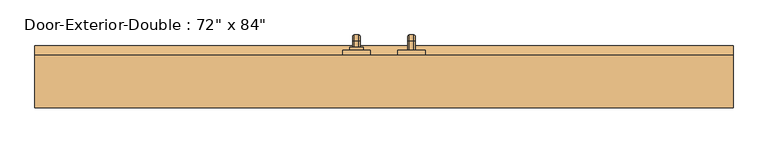
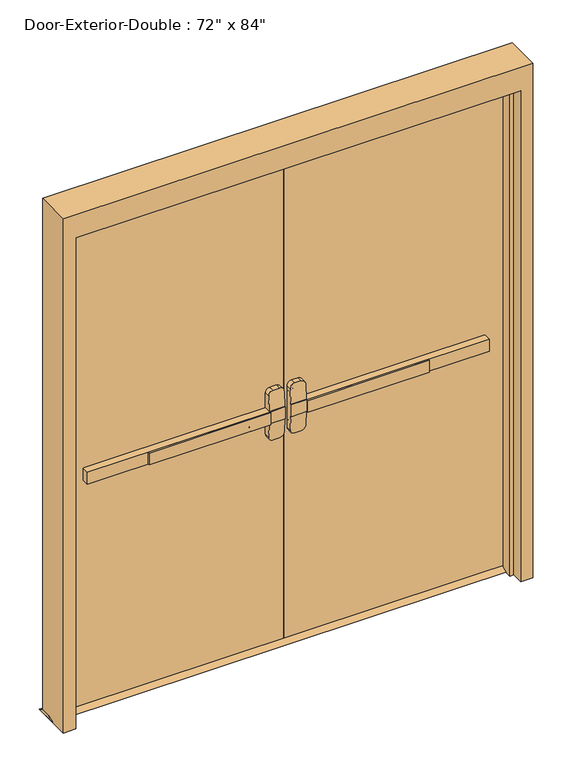
"""IFC4 building model written with IfcOpenShell, lengths in millimetres: door geometry."""

from ifc_helpers import new_model, si_unit, point, frame, frame_2d, origin, place, context, project, spatial, polyline, circle_curve, ellipse_curve, trimmed, segment, composite_curve, outline, extrude, faceted_brep, source, transform, mapped, element, save
from ifc_brep_helpers import plane_surface, cylinder_surface, revolved_surface, advanced_brep


def door_338a3df2(model_context):
    return source(origin(), model_context, "Body", "SolidModel", [
        extrude(outline(polyline([(-575.7333333, 11.1125), (-575.7333333, 17.4625), (-76.2, 17.4625), (-76.2, 11.1125), (-575.7333333, 11.1125)])), frame((0.0, 0.0, 990.6), z_axis=(0.0, 0.0, 1.0), x_axis=(1.0, 0.0, 0.0)), (0.0, 0.0, 1.0), 50.8),
        advanced_brep(
        [(-12.7, 17.4625, 1041.4), (-76.2, 17.4625, 1041.4), (-825.5, 17.4625, 1041.4), (-825.5, 17.4625, 990.6), (-76.2, 17.4625, 990.6), (-12.7, 17.4625, 990.6), (-825.5, 49.2125, 1041.4), (-76.2, 49.2125, 1041.4), (-76.2, 49.2125, 1104.9), (-57.15, 49.2125, 1123.95), (-31.75, 49.2125, 1123.95), (-12.7, 49.2125, 1104.9), (-12.7, 49.2125, 927.1), (-31.75, 49.2125, 908.05), (-57.15, 49.2125, 908.05), (-76.2, 49.2125, 927.1), (-76.2, 49.2125, 990.6), (-825.5, 49.2125, 990.6), (-12.7, 20.6377467, 1041.4), (-76.2, 20.6377467, 1041.4), (-12.7, 20.6377467, 990.6), (-12.7, 25.6479269, 927.1), (-12.7, 25.6479269, 1104.9), (-76.2, 20.6377467, 990.6), (-76.2, 25.6479269, 1104.9), (-76.2, 25.6479269, 927.1), (-57.15, 27.150981, 1123.95), (-31.75, 27.150981, 1123.95), (-31.75, 27.150981, 908.05), (-57.15, 27.150981, 908.05)],
        [
            (0, 1),
            (1, 2),
            (2, 3),
            (3, 4),
            (4, 5),
            (5, 0),
            (6, 7),
            (7, 8),
            (8, 9, circle_curve(frame((-57.15, 49.2125, 1104.9), z_axis=(0.0, 1.0, 0.0), x_axis=(-1.0, 0.0, 0.0)), 19.05)),
            (9, 10),
            (10, 11, circle_curve(frame((-31.75, 49.2125, 1104.9), z_axis=(0.0, 1.0, 0.0), x_axis=(-1.0, 0.0, 0.0)), 19.05)),
            (11, 12),
            (12, 13, circle_curve(frame((-31.75, 49.2125, 927.1), z_axis=(0.0, 1.0, 0.0), x_axis=(-1.0, 0.0, 0.0)), 19.05)),
            (13, 14),
            (14, 15, circle_curve(frame((-57.15, 49.2125, 927.1), z_axis=(0.0, 1.0, 0.0), x_axis=(-1.0, 0.0, 0.0)), 19.05)),
            (15, 16),
            (16, 17),
            (17, 6),
            (0, 18),
            (18, 19),
            (19, 7),
            (6, 2),
            (5, 20),
            (20, 21),
            (21, 12),
            (11, 22),
            (22, 18),
            (16, 23),
            (23, 20),
            (3, 17),
            (19, 24),
            (24, 8),
            (15, 25),
            (25, 23),
            (9, 26),
            (26, 27),
            (27, 10),
            (13, 28),
            (28, 29),
            (29, 14),
            (29, 25, ellipse_curve(frame((-57.15, 25.6479269, 927.1), z_axis=(0.0, 0.9969018152893365, 0.07865602756830282), x_axis=(0.0, -0.07865602756830208, 0.9969018152893365)), 19.1092038, 19.05)),
            (24, 26, ellipse_curve(frame((-57.15, 25.6479269, 1104.9), z_axis=(0.0, 0.9969018152893376, -0.07865602756828934), x_axis=(0.0, -0.078656027568288, -0.9969018152893377)), 19.1092038, 19.05)),
            (27, 22, ellipse_curve(frame((-31.75, 25.6479269, 1104.9), z_axis=(0.0, 0.9969018152893376, -0.07865602756828934), x_axis=(0.0, -0.078656027568288, -0.9969018152893377)), 19.1092038, 19.05)),
            (21, 28, ellipse_curve(frame((-31.75, 25.6479269, 927.1), z_axis=(0.0, 0.9969018152893365, 0.07865602756830282), x_axis=(0.0, -0.07865602756830208, 0.9969018152893365)), 19.1092038, 19.05)),
        ],
        [
            plane_surface(frame((-12.7, 17.4625, 1041.4), z_axis=(0.0, -1.0, 0.0), x_axis=(1.0, 0.0, 0.0))),
            plane_surface(frame((-12.7, 49.2125, 1041.4), z_axis=(0.0, 1.0, 0.0), x_axis=(-1.0, 0.0, 0.0))),
            plane_surface(frame((-825.5, 17.4625, 1041.4), z_axis=(0.0, 0.0, 1.0), x_axis=(0.0, 1.0, 0.0))),
            plane_surface(frame((-12.7, 17.4625, 1041.4), z_axis=(1.0, 0.0, 0.0), x_axis=(0.0, 1.0, 0.0))),
            plane_surface(frame((-12.7, 17.4625, 990.6), z_axis=(0.0, 0.0, -1.0), x_axis=(0.0, 1.0, 0.0))),
            plane_surface(frame((-825.5, 17.4625, 990.6), z_axis=(-1.0, 0.0, 0.0), x_axis=(0.0, 1.0, 0.0))),
            plane_surface(frame((-76.2, 20.6377467, 927.1), z_axis=(-1.0, 0.0, 0.0), x_axis=(0.0, 1.0, 0.0))),
            plane_surface(frame((-57.15, 20.6377467, 1123.95), z_axis=(0.0, 0.0, 1.0), x_axis=(0.0, 1.0, 0.0))),
            plane_surface(frame((-31.75, 20.6377467, 908.05), z_axis=(0.0, 0.0, -1.0), x_axis=(0.0, 1.0, 0.0))),
            cylinder_surface(frame((-57.15, 49.2125, 927.1), z_axis=(0.0, -1.0, 0.0), x_axis=(-1.0, 0.0, 0.0)), 19.05),
            cylinder_surface(frame((-57.15, 49.2125, 1104.9), z_axis=(0.0, -1.0, 0.0), x_axis=(-1.0, 0.0, 0.0)), 19.05),
            cylinder_surface(frame((-31.75, 49.2125, 1104.9), z_axis=(0.0, -1.0, 0.0), x_axis=(-1.0, 0.0, 0.0)), 19.05),
            cylinder_surface(frame((-31.75, 49.2125, 927.1), z_axis=(0.0, -1.0, 0.0), x_axis=(-1.0, 0.0, 0.0)), 19.05),
            plane_surface(frame((-76.2, 20.6377467, 1041.4), z_axis=(0.0, -0.9969018152893376, 0.07865602756828934), x_axis=(1.0, 0.0, 0.0))),
            plane_surface(frame((-76.2, 27.150981, 908.05), z_axis=(0.0, -0.9969018152893365, -0.07865602756830282), x_axis=(1.0, 0.0, 0.0))),
        ],
        [
            (0, [[1, 2, 3, 4, 5, 6]]),
            (1, [[7, 8, 9, 10, 11, 12, 13, 14, 15, 16, 17, 18]]),
            (2, [[-2, -1, 19, 20, 21, -7, 22]]),
            (3, [[23, 24, 25, -12, 26, 27, -19, -6]]),
            (4, [[-17, 28, 29, -23, -5, -4, 30]]),
            (5, [[-22, -18, -30, -3]]),
            (6, [[-21, 31, 32, -8]]),
            (6, [[33, 34, -28, -16]]),
            (7, [[35, 36, 37, -10]]),
            (8, [[38, 39, 40, -14]]),
            (9, [[-40, 41, -33, -15]]),
            (10, [[-32, 42, -35, -9]]),
            (11, [[-37, 43, -26, -11]]),
            (12, [[-25, 44, -38, -13]]),
            (13, [[-27, -43, -36, -42, -31, -20]]),
            (14, [[-29, -34, -41, -39, -44, -24]]),
        ],
    ),
        extrude(outline(polyline([(93.6625, 12.7), (119.0625, 0.0), (23.8125, 0.0), (49.2125, 12.7), (93.6625, 12.7)])), frame((-965.2, 0.0, 0.0), z_axis=(1.0, 0.0, 0.0), x_axis=(0.0, 1.0, 0.0)), (0.0, 0.0, 1.0), 1930.4),
        extrude(outline(polyline([(575.7333333, 11.1125), (76.2, 11.1125), (76.2, 17.4625), (575.7333333, 17.4625), (575.7333333, 11.1125)])), frame((0.0, 0.0, 990.6), z_axis=(0.0, 0.0, 1.0), x_axis=(1.0, 0.0, 0.0)), (0.0, 0.0, 1.0), 50.8),
        advanced_brep(
        [(12.7, 17.4625, 1041.4), (12.7, 17.4625, 990.6), (76.2, 17.4625, 990.6), (825.5, 17.4625, 990.6), (825.5, 17.4625, 1041.4), (76.2, 17.4625, 1041.4), (825.5, 49.2125, 1041.4), (825.5, 49.2125, 990.6), (76.2, 49.2125, 990.6), (76.2, 49.2125, 927.1), (57.15, 49.2125, 908.05), (31.75, 49.2125, 908.05), (12.7, 49.2125, 927.1), (12.7, 49.2125, 1104.9), (31.75, 49.2125, 1123.95), (57.15, 49.2125, 1123.95), (76.2, 49.2125, 1104.9), (76.2, 49.2125, 1041.4), (76.2, 20.6377467, 1041.4), (12.7, 20.6377467, 1041.4), (12.7, 25.6479269, 1104.9), (12.7, 25.6479269, 927.1), (12.7, 20.6377467, 990.6), (76.2, 20.6377467, 990.6), (76.2, 25.6479269, 927.1), (76.2, 25.6479269, 1104.9), (31.75, 27.150981, 1123.95), (57.15, 27.150981, 1123.95), (57.15, 27.150981, 908.05), (31.75, 27.150981, 908.05)],
        [
            (0, 1),
            (1, 2),
            (2, 3),
            (3, 4),
            (4, 5),
            (5, 0),
            (6, 7),
            (7, 8),
            (8, 9),
            (9, 10, circle_curve(frame((57.15, 49.2125, 927.1), z_axis=(0.0, 1.0, 0.0), x_axis=(1.0, 0.0, 0.0)), 19.05)),
            (10, 11),
            (11, 12, circle_curve(frame((31.75, 49.2125, 927.1), z_axis=(0.0, 1.0, 0.0), x_axis=(1.0, 0.0, 0.0)), 19.05)),
            (12, 13),
            (13, 14, circle_curve(frame((31.75, 49.2125, 1104.9), z_axis=(0.0, 1.0, 0.0), x_axis=(1.0, 0.0, 0.0)), 19.05)),
            (14, 15),
            (15, 16, circle_curve(frame((57.15, 49.2125, 1104.9), z_axis=(0.0, 1.0, 0.0), x_axis=(1.0, 0.0, 0.0)), 19.05)),
            (16, 17),
            (17, 6),
            (4, 6),
            (17, 18),
            (18, 19),
            (19, 0),
            (19, 20),
            (20, 13),
            (12, 21),
            (21, 22),
            (22, 1),
            (7, 3),
            (22, 23),
            (23, 8),
            (23, 24),
            (24, 9),
            (16, 25),
            (25, 18),
            (14, 26),
            (26, 27),
            (27, 15),
            (10, 28),
            (28, 29),
            (29, 11),
            (24, 28, ellipse_curve(frame((57.15, 25.6479269, 927.1), z_axis=(0.0, 0.9969018152893365, 0.07865602756830282), x_axis=(0.0, -0.07865602756830208, 0.9969018152893365)), 19.1092038, 19.05)),
            (27, 25, ellipse_curve(frame((57.15, 25.6479269, 1104.9), z_axis=(0.0, 0.9969018152893376, -0.07865602756828934), x_axis=(0.0, -0.078656027568288, -0.9969018152893377)), 19.1092038, 19.05)),
            (20, 26, ellipse_curve(frame((31.75, 25.6479269, 1104.9), z_axis=(0.0, 0.9969018152893376, -0.07865602756828934), x_axis=(0.0, -0.078656027568288, -0.9969018152893377)), 19.1092038, 19.05)),
            (29, 21, ellipse_curve(frame((31.75, 25.6479269, 927.1), z_axis=(0.0, 0.9969018152893365, 0.07865602756830282), x_axis=(0.0, -0.07865602756830208, 0.9969018152893365)), 19.1092038, 19.05)),
        ],
        [
            plane_surface(frame((12.7, 17.4625, 1041.4), z_axis=(0.0, -1.0, 0.0), x_axis=(-1.0, 0.0, 0.0))),
            plane_surface(frame((12.7, 49.2125, 1041.4), z_axis=(0.0, 1.0, 0.0), x_axis=(1.0, 0.0, 0.0))),
            plane_surface(frame((825.5, 17.4625, 1041.4), z_axis=(0.0, 0.0, 1.0), x_axis=(0.0, 1.0, 0.0))),
            plane_surface(frame((12.7, 17.4625, 1041.4), z_axis=(-1.0, 0.0, 0.0), x_axis=(0.0, 1.0, 0.0))),
            plane_surface(frame((12.7, 17.4625, 990.6), z_axis=(0.0, 0.0, -1.0), x_axis=(0.0, 1.0, 0.0))),
            plane_surface(frame((825.5, 17.4625, 990.6), z_axis=(1.0, 0.0, 0.0), x_axis=(0.0, 1.0, 0.0))),
            plane_surface(frame((76.2, 20.6377467, 927.1), z_axis=(1.0, 0.0, 0.0), x_axis=(0.0, 1.0, 0.0))),
            plane_surface(frame((57.15, 20.6377467, 1123.95), z_axis=(0.0, 0.0, 1.0), x_axis=(0.0, 1.0, 0.0))),
            plane_surface(frame((31.75, 20.6377467, 908.05), z_axis=(0.0, 0.0, -1.0), x_axis=(0.0, 1.0, 0.0))),
            cylinder_surface(frame((57.15, 49.2125, 927.1), z_axis=(0.0, -1.0, 0.0), x_axis=(1.0, 0.0, 0.0)), 19.05),
            cylinder_surface(frame((57.15, 49.2125, 1104.9), z_axis=(0.0, -1.0, 0.0), x_axis=(1.0, 0.0, 0.0)), 19.05),
            cylinder_surface(frame((31.75, 49.2125, 1104.9), z_axis=(0.0, -1.0, 0.0), x_axis=(1.0, 0.0, 0.0)), 19.05),
            cylinder_surface(frame((31.75, 49.2125, 927.1), z_axis=(0.0, -1.0, 0.0), x_axis=(1.0, 0.0, 0.0)), 19.05),
            plane_surface(frame((76.2, 20.6377467, 1041.4), z_axis=(0.0, -0.9969018152893376, 0.07865602756828934), x_axis=(-1.0, 0.0, 0.0))),
            plane_surface(frame((76.2, 27.150981, 908.05), z_axis=(0.0, -0.9969018152893365, -0.07865602756830282), x_axis=(-1.0, 0.0, 0.0))),
        ],
        [
            (0, [[1, 2, 3, 4, 5, 6]]),
            (1, [[7, 8, 9, 10, 11, 12, 13, 14, 15, 16, 17, 18]]),
            (2, [[19, -18, 20, 21, 22, -6, -5]]),
            (3, [[-1, -22, 23, 24, -13, 25, 26, 27]]),
            (4, [[28, -3, -2, -27, 29, 30, -8]]),
            (5, [[-4, -28, -7, -19]]),
            (6, [[-9, -30, 31, 32]]),
            (6, [[-17, 33, 34, -20]]),
            (7, [[-15, 35, 36, 37]]),
            (8, [[-11, 38, 39, 40]]),
            (9, [[-10, -32, 41, -38]]),
            (10, [[-16, -37, 42, -33]]),
            (11, [[-14, -24, 43, -35]]),
            (12, [[-12, -40, 44, -25]]),
            (13, [[-21, -34, -42, -36, -43, -23]]),
            (14, [[-26, -44, -39, -41, -31, -29]]),
        ],
    ),
        advanced_brep(
        [(66.2, 106.3625, 1017.190625), (66.2, 106.3625, 1014.809375), (69.771875, 106.3625, 1011.2375), (82.6284594, 106.3625, 1011.2375), (86.2, 106.3625, 1014.8090406), (86.2, 106.3625, 1017.190625), (82.628125, 106.3625, 1020.7625), (69.771875, 106.3625, 1020.7625), (66.2, 106.3625, 887.809375), (69.771875, 106.3625, 884.2375), (82.628125, 106.3625, 884.2375), (86.2, 106.3625, 887.809375), (86.2, 106.3625, 890.1909594), (82.6284594, 106.3625, 893.7625), (69.771875, 106.3625, 893.7625), (66.2, 106.3625, 890.190625), (66.2, 131.7625, 1017.190625), (66.2, 145.653125, 1003.3), (66.2, 145.653125, 901.7), (66.2, 131.7625, 887.809375), (66.2, 131.7625, 890.190625), (66.2, 143.271875, 901.7), (66.2, 143.271875, 1003.3), (66.2, 131.7625, 1014.809375), (69.771875, 131.7625, 1011.2375), (82.6284594, 131.7625, 1011.2375), (86.2, 131.7625, 1014.8090406), (86.2, 143.2715406, 1003.3), (86.2, 143.2715406, 901.7), (86.2, 131.7625, 890.1909594), (86.2, 131.7625, 887.809375), (86.2, 145.653125, 901.7), (86.2, 145.653125, 1003.3), (86.2, 131.7625, 1017.190625), (82.628125, 131.7625, 1020.7625), (69.771875, 131.7625, 1020.7625), (69.771875, 139.7, 1003.3), (82.6284594, 139.7, 1003.3), (82.628125, 149.225, 1003.3), (69.771875, 149.225, 1003.3), (69.771875, 139.7, 901.7), (82.6284594, 139.7, 901.7), (82.628125, 149.225, 901.7), (69.771875, 149.225, 901.7), (69.771875, 131.7625, 893.7625), (82.6284594, 131.7625, 893.7625), (82.628125, 131.7625, 884.2375), (69.771875, 131.7625, 884.2375)],
        [
            (0, 1),
            (1, 2, circle_curve(frame((69.771875, 106.3625, 1014.809375), z_axis=(0.0, -1.0, 0.0), x_axis=(0.0, 0.0, 1.0)), 3.571875)),
            (2, 3),
            (3, 4, circle_curve(frame((82.6284594, 106.3625, 1014.8090406), z_axis=(0.0, -1.0, 0.0), x_axis=(0.0, 0.0, 1.0)), 3.5715406)),
            (4, 5),
            (5, 6, circle_curve(frame((82.628125, 106.3625, 1017.190625), z_axis=(0.0, -1.0, 0.0), x_axis=(0.0, 0.0, 1.0)), 3.571875)),
            (6, 7),
            (7, 0, circle_curve(frame((69.771875, 106.3625, 1017.190625), z_axis=(0.0, -1.0, 0.0), x_axis=(0.0, 0.0, 1.0)), 3.571875)),
            (8, 9, circle_curve(frame((69.771875, 106.3625, 887.809375), z_axis=(0.0, -1.0, 0.0), x_axis=(0.0, 0.0, -1.0)), 3.571875)),
            (9, 10),
            (10, 11, circle_curve(frame((82.628125, 106.3625, 887.809375), z_axis=(0.0, -1.0, 0.0), x_axis=(0.0, 0.0, -1.0)), 3.571875)),
            (11, 12),
            (12, 13, circle_curve(frame((82.6284594, 106.3625, 890.1909594), z_axis=(0.0, -1.0, 0.0), x_axis=(0.0, 0.0, -1.0)), 3.5715406)),
            (13, 14),
            (14, 15, circle_curve(frame((69.771875, 106.3625, 890.190625), z_axis=(0.0, -1.0, 0.0), x_axis=(0.0, 0.0, -1.0)), 3.571875)),
            (15, 8),
            (0, 16),
            (16, 17, circle_curve(frame((66.2, 131.7625, 1003.3), z_axis=(-1.0, 0.0, 0.0), x_axis=(0.0, 0.0, 1.0)), 13.890625)),
            (17, 18),
            (18, 19, circle_curve(frame((66.2, 131.7625, 901.7), z_axis=(-1.0, 0.0, 0.0), x_axis=(0.0, 1.0, 0.0)), 13.890625)),
            (19, 8),
            (15, 20),
            (20, 21, circle_curve(frame((66.2, 131.7625, 901.7), z_axis=(1.0, 0.0, 0.0), x_axis=(0.0, 1.0, 0.0)), 11.509375)),
            (21, 22),
            (22, 23, circle_curve(frame((66.2, 131.7625, 1003.3), z_axis=(1.0, 0.0, 0.0), x_axis=(0.0, 0.0, 1.0)), 11.509375)),
            (23, 1),
            (23, 24, circle_curve(frame((69.771875, 131.7625, 1014.809375), z_axis=(0.0, -1.0, 0.0), x_axis=(0.0, 0.0, 1.0)), 3.571875)),
            (24, 2),
            (24, 25),
            (25, 3),
            (25, 26, circle_curve(frame((82.6284594, 131.7625, 1014.8090406), z_axis=(0.0, -1.0, 0.0), x_axis=(0.0, 0.0, 1.0)), 3.5715406)),
            (26, 4),
            (26, 27, circle_curve(frame((86.2, 131.7625, 1003.3), z_axis=(-1.0, 0.0, 0.0), x_axis=(0.0, 0.0, 1.0)), 11.5090406)),
            (27, 28),
            (28, 29, circle_curve(frame((86.2, 131.7625, 901.7), z_axis=(-1.0, 0.0, 0.0), x_axis=(0.0, 1.0, 0.0)), 11.5090406)),
            (29, 12),
            (11, 30),
            (30, 31, circle_curve(frame((86.2, 131.7625, 901.7), z_axis=(1.0, 0.0, 0.0), x_axis=(0.0, 1.0, 0.0)), 13.890625)),
            (31, 32),
            (32, 33, circle_curve(frame((86.2, 131.7625, 1003.3), z_axis=(1.0, 0.0, 0.0), x_axis=(0.0, 0.0, 1.0)), 13.890625)),
            (33, 5),
            (33, 34, circle_curve(frame((82.628125, 131.7625, 1017.190625), z_axis=(0.0, -1.0, 0.0), x_axis=(0.0, 0.0, 1.0)), 3.571875)),
            (34, 6),
            (34, 35),
            (35, 7),
            (35, 16, circle_curve(frame((69.771875, 131.7625, 1017.190625), z_axis=(0.0, -1.0, 0.0), x_axis=(0.0, 0.0, 1.0)), 3.571875)),
            (36, 24, circle_curve(frame((69.771875, 131.7625, 1003.3), z_axis=(1.0, 0.0, 0.0), x_axis=(0.0, 0.0, 1.0)), 7.9375)),
            (22, 36, circle_curve(frame((69.771875, 143.271875, 1003.3), z_axis=(0.0, 0.0, 1.0), x_axis=(0.0, 1.0, 0.0)), 3.571875)),
            (37, 25, circle_curve(frame((82.6284594, 131.7625, 1003.3), z_axis=(1.0, 0.0, 0.0), x_axis=(0.0, 0.0, 1.0)), 7.9375)),
            (36, 37),
            (37, 27, circle_curve(frame((82.6284594, 143.2715406, 1003.3), z_axis=(0.0, 0.0, 1.0), x_axis=(0.0, 1.0, 0.0)), 3.5715406)),
            (38, 34, circle_curve(frame((82.628125, 131.7625, 1003.3), z_axis=(1.0, 0.0, 0.0), x_axis=(0.0, 0.0, 1.0)), 17.4625)),
            (32, 38, circle_curve(frame((82.628125, 145.653125, 1003.3), z_axis=(0.0, 0.0, 1.0), x_axis=(0.0, 1.0, 0.0)), 3.571875)),
            (39, 35, circle_curve(frame((69.771875, 131.7625, 1003.3), z_axis=(1.0, 0.0, 0.0), x_axis=(0.0, 0.0, 1.0)), 17.4625)),
            (38, 39),
            (39, 17, circle_curve(frame((69.771875, 145.653125, 1003.3), z_axis=(0.0, 0.0, 1.0), x_axis=(0.0, 1.0, 0.0)), 3.571875)),
            (21, 40, circle_curve(frame((69.771875, 143.271875, 901.7), z_axis=(0.0, 0.0, 1.0), x_axis=(0.0, 1.0, 0.0)), 3.571875)),
            (40, 36),
            (40, 41),
            (41, 37),
            (41, 28, circle_curve(frame((82.6284594, 143.2715406, 901.7), z_axis=(0.0, 0.0, 1.0), x_axis=(0.0, 1.0, 0.0)), 3.5715406)),
            (31, 42, circle_curve(frame((82.628125, 145.653125, 901.7), z_axis=(0.0, 0.0, 1.0), x_axis=(0.0, 1.0, 0.0)), 3.571875)),
            (42, 38),
            (42, 43),
            (43, 39),
            (43, 18, circle_curve(frame((69.771875, 145.653125, 901.7), z_axis=(0.0, 0.0, 1.0), x_axis=(0.0, 1.0, 0.0)), 3.571875)),
            (44, 40, circle_curve(frame((69.771875, 131.7625, 901.7), z_axis=(1.0, 0.0, 0.0), x_axis=(0.0, 1.0, 0.0)), 7.9375)),
            (20, 44, circle_curve(frame((69.771875, 131.7625, 890.190625), z_axis=(0.0, 1.0, 0.0), x_axis=(0.0, 0.0, -1.0)), 3.571875)),
            (45, 41, circle_curve(frame((82.6284594, 131.7625, 901.7), z_axis=(1.0, 0.0, 0.0), x_axis=(0.0, 1.0, 0.0)), 7.9375)),
            (44, 45),
            (45, 29, circle_curve(frame((82.6284594, 131.7625, 890.1909594), z_axis=(0.0, 1.0, 0.0), x_axis=(0.0, 0.0, -1.0)), 3.5715406)),
            (46, 42, circle_curve(frame((82.628125, 131.7625, 901.7), z_axis=(1.0, 0.0, 0.0), x_axis=(0.0, 1.0, 0.0)), 17.4625)),
            (30, 46, circle_curve(frame((82.628125, 131.7625, 887.809375), z_axis=(0.0, 1.0, 0.0), x_axis=(0.0, 0.0, -1.0)), 3.571875)),
            (47, 43, circle_curve(frame((69.771875, 131.7625, 901.7), z_axis=(1.0, 0.0, 0.0), x_axis=(0.0, 1.0, 0.0)), 17.4625)),
            (46, 47),
            (47, 19, circle_curve(frame((69.771875, 131.7625, 887.809375), z_axis=(0.0, 1.0, 0.0), x_axis=(0.0, 0.0, -1.0)), 3.571875)),
            (14, 44),
            (13, 45),
            (10, 46),
            (9, 47),
        ],
        [
            plane_surface(frame((76.2, 106.3625, 1016.0), z_axis=(0.0, -1.0, 0.0), x_axis=(1.0, 0.0, 0.0))),
            plane_surface(frame((76.2, 106.3625, 889.0), z_axis=(0.0, -1.0, 0.0), x_axis=(1.0, 0.0, 0.0))),
            plane_surface(frame((66.2, 106.3625, 1017.190625), z_axis=(-1.0, 0.0, 0.0), x_axis=(0.0, 1.0, 0.0))),
            cylinder_surface(frame((69.771875, 106.3625, 1014.809375), z_axis=(0.0, -1.0, 0.0), x_axis=(0.0, 0.0, 1.0)), 3.571875),
            plane_surface(frame((69.771875, 106.3625, 1011.2375), z_axis=(0.0, 0.0, -1.0), x_axis=(0.0, 1.0, 0.0))),
            cylinder_surface(frame((82.6284594, 106.3625, 1014.8090406), z_axis=(0.0, -1.0, 0.0), x_axis=(0.0, 0.0, 1.0)), 3.5715406),
            plane_surface(frame((86.2, 106.3625, 1014.8090406), z_axis=(1.0, 0.0, 0.0), x_axis=(0.0, 1.0, 0.0))),
            cylinder_surface(frame((82.628125, 106.3625, 1017.190625), z_axis=(0.0, -1.0, 0.0), x_axis=(0.0, 0.0, 1.0)), 3.571875),
            plane_surface(frame((82.628125, 106.3625, 1020.7625), z_axis=(0.0, 0.0, 1.0), x_axis=(0.0, 1.0, 0.0))),
            cylinder_surface(frame((69.771875, 106.3625, 1017.190625), z_axis=(0.0, -1.0, 0.0), x_axis=(0.0, 0.0, 1.0)), 3.571875),
            revolved_surface(trimmed(ellipse_curve(frame((69.771875, 131.7625, 1014.809375), z_axis=(0.0, -1.0, 0.0), x_axis=(0.0, 0.0, 1.0)), 3.571875, 3.571875), [point((66.2, 131.7625, 1014.809375))], [point((69.771875, 131.7625, 1011.2375))], True, "CARTESIAN"), (76.2, 131.7625, 1003.3), (-1.0, 0.0, 0.0)),
            revolved_surface(polyline([(69.771875, 131.7625, 1011.2375), (82.6284594, 131.7625, 1011.2375)]), (76.2, 131.7625, 1003.3), (-1.0, 0.0, 0.0)),
            revolved_surface(trimmed(ellipse_curve(frame((82.6284594, 131.7625, 1014.8090406), z_axis=(0.0, -1.0, 0.0), x_axis=(0.0, 0.0, 1.0)), 3.5715406, 3.5715406), [point((82.6284594, 131.7625, 1011.2375))], [point((86.2, 131.7625, 1014.8090406))], True, "CARTESIAN"), (76.2, 131.7625, 1003.3), (-1.0, 0.0, 0.0)),
            revolved_surface(trimmed(ellipse_curve(frame((82.628125, 131.7625, 1017.190625), z_axis=(0.0, -1.0, 0.0), x_axis=(0.0, 0.0, 1.0)), 3.571875, 3.571875), [point((86.2, 131.7625, 1017.190625))], [point((82.628125, 131.7625, 1020.7625))], True, "CARTESIAN"), (76.2, 131.7625, 1003.3), (-1.0, 0.0, 0.0)),
            cylinder_surface(frame((76.2, 131.7625, 1003.3), z_axis=(-1.0, 0.0, 0.0), x_axis=(0.0, 0.0, 1.0)), 17.4625),
            revolved_surface(trimmed(ellipse_curve(frame((69.771875, 131.7625, 1017.190625), z_axis=(0.0, -1.0, 0.0), x_axis=(0.0, 0.0, 1.0)), 3.571875, 3.571875), [point((69.771875, 131.7625, 1020.7625))], [point((66.2, 131.7625, 1017.190625))], True, "CARTESIAN"), (76.2, 131.7625, 1003.3), (-1.0, 0.0, 0.0)),
            cylinder_surface(frame((69.771875, 143.271875, 1003.3), z_axis=(0.0, 0.0, 1.0), x_axis=(0.0, 1.0, 0.0)), 3.571875),
            plane_surface(frame((69.771875, 139.7, 1003.3), z_axis=(0.0, -1.0, 0.0), x_axis=(0.0, 0.0, -1.0))),
            cylinder_surface(frame((82.6284594, 143.2715406, 1003.3), z_axis=(0.0, 0.0, 1.0), x_axis=(0.0, 1.0, 0.0)), 3.5715406),
            cylinder_surface(frame((82.628125, 145.653125, 1003.3), z_axis=(0.0, 0.0, 1.0), x_axis=(0.0, 1.0, 0.0)), 3.571875),
            plane_surface(frame((82.628125, 149.225, 1003.3), z_axis=(0.0, 1.0, 0.0), x_axis=(0.0, 0.0, -1.0))),
            cylinder_surface(frame((69.771875, 145.653125, 1003.3), z_axis=(0.0, 0.0, 1.0), x_axis=(0.0, 1.0, 0.0)), 3.571875),
            revolved_surface(trimmed(ellipse_curve(frame((69.771875, 143.271875, 901.7), z_axis=(0.0, 0.0, 1.0), x_axis=(0.0, 1.0, 0.0)), 3.571875, 3.571875), [point((66.2, 143.271875, 901.7))], [point((69.771875, 139.7, 901.7))], True, "CARTESIAN"), (76.2, 131.7625, 901.7), (-1.0, 0.0, 0.0)),
            revolved_surface(polyline([(69.771875, 139.7, 901.7), (82.6284594, 139.7, 901.7)]), (76.2, 131.7625, 901.7), (-1.0, 0.0, 0.0)),
            revolved_surface(trimmed(ellipse_curve(frame((82.6284594, 143.2715406, 901.7), z_axis=(0.0, 0.0, 1.0), x_axis=(0.0, 1.0, 0.0)), 3.5715406, 3.5715406), [point((82.6284594, 139.7, 901.7))], [point((86.2, 143.2715406, 901.7))], True, "CARTESIAN"), (76.2, 131.7625, 901.7), (-1.0, 0.0, 0.0)),
            revolved_surface(trimmed(ellipse_curve(frame((82.628125, 145.653125, 901.7), z_axis=(0.0, 0.0, 1.0), x_axis=(0.0, 1.0, 0.0)), 3.571875, 3.571875), [point((86.2, 145.653125, 901.7))], [point((82.628125, 149.225, 901.7))], True, "CARTESIAN"), (76.2, 131.7625, 901.7), (-1.0, 0.0, 0.0)),
            cylinder_surface(frame((76.2, 131.7625, 901.7), z_axis=(-1.0, 0.0, 0.0), x_axis=(0.0, 1.0, 0.0)), 17.4625),
            revolved_surface(trimmed(ellipse_curve(frame((69.771875, 145.653125, 901.7), z_axis=(0.0, 0.0, 1.0), x_axis=(0.0, 1.0, 0.0)), 3.571875, 3.571875), [point((69.771875, 149.225, 901.7))], [point((66.2, 145.653125, 901.7))], True, "CARTESIAN"), (76.2, 131.7625, 901.7), (-1.0, 0.0, 0.0)),
            cylinder_surface(frame((69.771875, 131.7625, 890.190625), z_axis=(0.0, 1.0, 0.0), x_axis=(0.0, 0.0, -1.0)), 3.571875),
            plane_surface(frame((69.771875, 131.7625, 893.7625), z_axis=(0.0, 0.0, 1.0), x_axis=(0.0, -1.0, 0.0))),
            cylinder_surface(frame((82.6284594, 131.7625, 890.1909594), z_axis=(0.0, 1.0, 0.0), x_axis=(0.0, 0.0, -1.0)), 3.5715406),
            cylinder_surface(frame((82.628125, 131.7625, 887.809375), z_axis=(0.0, 1.0, 0.0), x_axis=(0.0, 0.0, -1.0)), 3.571875),
            plane_surface(frame((82.628125, 131.7625, 884.2375), z_axis=(0.0, 0.0, -1.0), x_axis=(0.0, -1.0, 0.0))),
            cylinder_surface(frame((69.771875, 131.7625, 887.809375), z_axis=(0.0, 1.0, 0.0), x_axis=(0.0, 0.0, -1.0)), 3.571875),
        ],
        [
            (0, [[1, 2, 3, 4, 5, 6, 7, 8]]),
            (1, [[9, 10, 11, 12, 13, 14, 15, 16]]),
            (2, [[-1, 17, 18, 19, 20, 21, -16, 22, 23, 24, 25, 26]]),
            (3, [[-2, -26, 27, 28]]),
            (4, [[-3, -28, 29, 30]]),
            (5, [[-4, -30, 31, 32]]),
            (6, [[-5, -32, 33, 34, 35, 36, -12, 37, 38, 39, 40, 41]]),
            (7, [[-6, -41, 42, 43]]),
            (8, [[-7, -43, 44, 45]]),
            (9, [[-8, -45, 46, -17]]),
            (10, [[47, -27, -25, 48]]),
            (11, [[49, -29, -47, 50]]),
            (12, [[-33, -31, -49, 51]]),
            (13, [[52, -42, -40, 53]]),
            (14, [[54, -44, -52, 55]]),
            (15, [[-18, -46, -54, 56]]),
            (16, [[-48, -24, 57, 58]]),
            (17, [[-50, -58, 59, 60]]),
            (18, [[-51, -60, 61, -34]]),
            (19, [[-53, -39, 62, 63]]),
            (20, [[-55, -63, 64, 65]]),
            (21, [[-56, -65, 66, -19]]),
            (22, [[67, -57, -23, 68]]),
            (23, [[69, -59, -67, 70]]),
            (24, [[-35, -61, -69, 71]]),
            (25, [[72, -62, -38, 73]]),
            (26, [[74, -64, -72, 75]]),
            (27, [[-20, -66, -74, 76]]),
            (28, [[-68, -22, -15, 77]]),
            (29, [[-70, -77, -14, 78]]),
            (30, [[-71, -78, -13, -36]]),
            (31, [[-73, -37, -11, 79]]),
            (32, [[-75, -79, -10, 80]]),
            (33, [[-76, -80, -9, -21]]),
        ],
    ),
        extrude(outline(composite_curve([segment(trimmed(circle_curve(frame_2d((1113.0338574, 76.2)), 89.3016225), [point((1193.8, 114.3))], [point((1193.8, 38.1))], False, "CARTESIAN"), True, "CONTINUOUS"), segment(polyline([(1193.8, 38.1), (838.2, 38.1)]), True, "CONTINUOUS"), segment(trimmed(circle_curve(frame_2d((918.9661426, 76.2)), 89.3016225), [point((838.2, 38.1))], [point((838.2, 114.3))], False, "CARTESIAN"), True, "CONTINUOUS"), segment(polyline([(838.2, 114.3), (1193.8, 114.3)]), True, "CONTINUOUS")], self_intersect=False)), frame((0.0, 93.6625, 0.0), z_axis=(0.0, 1.0, 0.0), x_axis=(0.0, 0.0, 1.0)), (0.0, 0.0, 1.0), 12.7),
        advanced_brep(
        [(-86.2, 106.3625, 1017.190625), (-86.2, 106.3625, 1014.809375), (-82.628125, 106.3625, 1011.2375), (-69.7715406, 106.3625, 1011.2375), (-66.2, 106.3625, 1014.8090406), (-66.2, 106.3625, 1017.190625), (-69.771875, 106.3625, 1020.7625), (-82.628125, 106.3625, 1020.7625), (-86.2, 106.3625, 887.809375), (-82.628125, 106.3625, 884.2375), (-69.771875, 106.3625, 884.2375), (-66.2, 106.3625, 887.809375), (-66.2, 106.3625, 890.1909594), (-69.7715406, 106.3625, 893.7625), (-82.628125, 106.3625, 893.7625), (-86.2, 106.3625, 890.190625), (-86.2, 131.7625, 1017.190625), (-86.2, 145.653125, 1003.3), (-86.2, 145.653125, 901.7), (-86.2, 131.7625, 887.809375), (-86.2, 131.7625, 890.190625), (-86.2, 143.271875, 901.7), (-86.2, 143.271875, 1003.3), (-86.2, 131.7625, 1014.809375), (-82.628125, 131.7625, 1011.2375), (-69.7715406, 131.7625, 1011.2375), (-66.2, 131.7625, 1014.8090406), (-66.2, 143.2715406, 1003.3), (-66.2, 143.2715406, 901.7), (-66.2, 131.7625, 890.1909594), (-66.2, 131.7625, 887.809375), (-66.2, 145.653125, 901.7), (-66.2, 145.653125, 1003.3), (-66.2, 131.7625, 1017.190625), (-69.771875, 131.7625, 1020.7625), (-82.628125, 131.7625, 1020.7625), (-82.628125, 139.7, 1003.3), (-69.7715406, 139.7, 1003.3), (-69.771875, 149.225, 1003.3), (-82.628125, 149.225, 1003.3), (-82.628125, 139.7, 901.7), (-69.7715406, 139.7, 901.7), (-69.771875, 149.225, 901.7), (-82.628125, 149.225, 901.7), (-82.628125, 131.7625, 893.7625), (-69.7715406, 131.7625, 893.7625), (-69.771875, 131.7625, 884.2375), (-82.628125, 131.7625, 884.2375)],
        [
            (0, 1),
            (1, 2, circle_curve(frame((-82.628125, 106.3625, 1014.809375), z_axis=(0.0, -1.0, 0.0), x_axis=(0.0, 0.0, 1.0)), 3.571875)),
            (2, 3),
            (3, 4, circle_curve(frame((-69.7715406, 106.3625, 1014.8090406), z_axis=(0.0, -1.0, 0.0), x_axis=(0.0, 0.0, 1.0)), 3.5715406)),
            (4, 5),
            (5, 6, circle_curve(frame((-69.771875, 106.3625, 1017.190625), z_axis=(0.0, -1.0, 0.0), x_axis=(0.0, 0.0, 1.0)), 3.571875)),
            (6, 7),
            (7, 0, circle_curve(frame((-82.628125, 106.3625, 1017.190625), z_axis=(0.0, -1.0, 0.0), x_axis=(0.0, 0.0, 1.0)), 3.571875)),
            (8, 9, circle_curve(frame((-82.628125, 106.3625, 887.809375), z_axis=(0.0, -1.0, 0.0), x_axis=(0.0, 0.0, -1.0)), 3.571875)),
            (9, 10),
            (10, 11, circle_curve(frame((-69.771875, 106.3625, 887.809375), z_axis=(0.0, -1.0, 0.0), x_axis=(0.0, 0.0, -1.0)), 3.571875)),
            (11, 12),
            (12, 13, circle_curve(frame((-69.7715406, 106.3625, 890.1909594), z_axis=(0.0, -1.0, 0.0), x_axis=(0.0, 0.0, -1.0)), 3.5715406)),
            (13, 14),
            (14, 15, circle_curve(frame((-82.628125, 106.3625, 890.190625), z_axis=(0.0, -1.0, 0.0), x_axis=(0.0, 0.0, -1.0)), 3.571875)),
            (15, 8),
            (0, 16),
            (16, 17, circle_curve(frame((-86.2, 131.7625, 1003.3), z_axis=(-1.0, 0.0, 0.0), x_axis=(0.0, 0.0, 1.0)), 13.890625)),
            (17, 18),
            (18, 19, circle_curve(frame((-86.2, 131.7625, 901.7), z_axis=(-1.0, 0.0, 0.0), x_axis=(0.0, 1.0, 0.0)), 13.890625)),
            (19, 8),
            (15, 20),
            (20, 21, circle_curve(frame((-86.2, 131.7625, 901.7), z_axis=(1.0, 0.0, 0.0), x_axis=(0.0, 1.0, 0.0)), 11.509375)),
            (21, 22),
            (22, 23, circle_curve(frame((-86.2, 131.7625, 1003.3), z_axis=(1.0, 0.0, 0.0), x_axis=(0.0, 0.0, 1.0)), 11.509375)),
            (23, 1),
            (23, 24, circle_curve(frame((-82.628125, 131.7625, 1014.809375), z_axis=(0.0, -1.0, 0.0), x_axis=(0.0, 0.0, 1.0)), 3.571875)),
            (24, 2),
            (24, 25),
            (25, 3),
            (25, 26, circle_curve(frame((-69.7715406, 131.7625, 1014.8090406), z_axis=(0.0, -1.0, 0.0), x_axis=(0.0, 0.0, 1.0)), 3.5715406)),
            (26, 4),
            (26, 27, circle_curve(frame((-66.2, 131.7625, 1003.3), z_axis=(-1.0, 0.0, 0.0), x_axis=(0.0, 0.0, 1.0)), 11.5090406)),
            (27, 28),
            (28, 29, circle_curve(frame((-66.2, 131.7625, 901.7), z_axis=(-1.0, 0.0, 0.0), x_axis=(0.0, 1.0, 0.0)), 11.5090406)),
            (29, 12),
            (11, 30),
            (30, 31, circle_curve(frame((-66.2, 131.7625, 901.7), z_axis=(1.0, 0.0, 0.0), x_axis=(0.0, 1.0, 0.0)), 13.890625)),
            (31, 32),
            (32, 33, circle_curve(frame((-66.2, 131.7625, 1003.3), z_axis=(1.0, 0.0, 0.0), x_axis=(0.0, 0.0, 1.0)), 13.890625)),
            (33, 5),
            (33, 34, circle_curve(frame((-69.771875, 131.7625, 1017.190625), z_axis=(0.0, -1.0, 0.0), x_axis=(0.0, 0.0, 1.0)), 3.571875)),
            (34, 6),
            (34, 35),
            (35, 7),
            (35, 16, circle_curve(frame((-82.628125, 131.7625, 1017.190625), z_axis=(0.0, -1.0, 0.0), x_axis=(0.0, 0.0, 1.0)), 3.571875)),
            (36, 24, circle_curve(frame((-82.628125, 131.7625, 1003.3), z_axis=(1.0, 0.0, 0.0), x_axis=(0.0, 0.0, 1.0)), 7.9375)),
            (22, 36, circle_curve(frame((-82.628125, 143.271875, 1003.3), z_axis=(0.0, 0.0, 1.0), x_axis=(0.0, 1.0, 0.0)), 3.571875)),
            (37, 25, circle_curve(frame((-69.7715406, 131.7625, 1003.3), z_axis=(1.0, 0.0, 0.0), x_axis=(0.0, 0.0, 1.0)), 7.9375)),
            (36, 37),
            (37, 27, circle_curve(frame((-69.7715406, 143.2715406, 1003.3), z_axis=(0.0, 0.0, 1.0), x_axis=(0.0, 1.0, 0.0)), 3.5715406)),
            (38, 34, circle_curve(frame((-69.771875, 131.7625, 1003.3), z_axis=(1.0, 0.0, 0.0), x_axis=(0.0, 0.0, 1.0)), 17.4625)),
            (32, 38, circle_curve(frame((-69.771875, 145.653125, 1003.3), z_axis=(0.0, 0.0, 1.0), x_axis=(0.0, 1.0, 0.0)), 3.571875)),
            (39, 35, circle_curve(frame((-82.628125, 131.7625, 1003.3), z_axis=(1.0, 0.0, 0.0), x_axis=(0.0, 0.0, 1.0)), 17.4625)),
            (38, 39),
            (39, 17, circle_curve(frame((-82.628125, 145.653125, 1003.3), z_axis=(0.0, 0.0, 1.0), x_axis=(0.0, 1.0, 0.0)), 3.571875)),
            (21, 40, circle_curve(frame((-82.628125, 143.271875, 901.7), z_axis=(0.0, 0.0, 1.0), x_axis=(0.0, 1.0, 0.0)), 3.571875)),
            (40, 36),
            (40, 41),
            (41, 37),
            (41, 28, circle_curve(frame((-69.7715406, 143.2715406, 901.7), z_axis=(0.0, 0.0, 1.0), x_axis=(0.0, 1.0, 0.0)), 3.5715406)),
            (31, 42, circle_curve(frame((-69.771875, 145.653125, 901.7), z_axis=(0.0, 0.0, 1.0), x_axis=(0.0, 1.0, 0.0)), 3.571875)),
            (42, 38),
            (42, 43),
            (43, 39),
            (43, 18, circle_curve(frame((-82.628125, 145.653125, 901.7), z_axis=(0.0, 0.0, 1.0), x_axis=(0.0, 1.0, 0.0)), 3.571875)),
            (44, 40, circle_curve(frame((-82.628125, 131.7625, 901.7), z_axis=(1.0, 0.0, 0.0), x_axis=(0.0, 1.0, 0.0)), 7.9375)),
            (20, 44, circle_curve(frame((-82.628125, 131.7625, 890.190625), z_axis=(0.0, 1.0, 0.0), x_axis=(0.0, 0.0, -1.0)), 3.571875)),
            (45, 41, circle_curve(frame((-69.7715406, 131.7625, 901.7), z_axis=(1.0, 0.0, 0.0), x_axis=(0.0, 1.0, 0.0)), 7.9375)),
            (44, 45),
            (45, 29, circle_curve(frame((-69.7715406, 131.7625, 890.1909594), z_axis=(0.0, 1.0, 0.0), x_axis=(0.0, 0.0, -1.0)), 3.5715406)),
            (46, 42, circle_curve(frame((-69.771875, 131.7625, 901.7), z_axis=(1.0, 0.0, 0.0), x_axis=(0.0, 1.0, 0.0)), 17.4625)),
            (30, 46, circle_curve(frame((-69.771875, 131.7625, 887.809375), z_axis=(0.0, 1.0, 0.0), x_axis=(0.0, 0.0, -1.0)), 3.571875)),
            (47, 43, circle_curve(frame((-82.628125, 131.7625, 901.7), z_axis=(1.0, 0.0, 0.0), x_axis=(0.0, 1.0, 0.0)), 17.4625)),
            (46, 47),
            (47, 19, circle_curve(frame((-82.628125, 131.7625, 887.809375), z_axis=(0.0, 1.0, 0.0), x_axis=(0.0, 0.0, -1.0)), 3.571875)),
            (14, 44),
            (13, 45),
            (10, 46),
            (9, 47),
        ],
        [
            plane_surface(frame((-76.2, 106.3625, 1016.0), z_axis=(0.0, -1.0, 0.0), x_axis=(1.0, 0.0, 0.0))),
            plane_surface(frame((-76.2, 106.3625, 889.0), z_axis=(0.0, -1.0, 0.0), x_axis=(1.0, 0.0, 0.0))),
            plane_surface(frame((-86.2, 106.3625, 1017.190625), z_axis=(-1.0, 0.0, 0.0), x_axis=(0.0, 1.0, 0.0))),
            cylinder_surface(frame((-82.628125, 106.3625, 1014.809375), z_axis=(0.0, -1.0, 0.0), x_axis=(0.0, 0.0, 1.0)), 3.571875),
            plane_surface(frame((-82.628125, 106.3625, 1011.2375), z_axis=(0.0, 0.0, -1.0), x_axis=(0.0, 1.0, 0.0))),
            cylinder_surface(frame((-69.7715406, 106.3625, 1014.8090406), z_axis=(0.0, -1.0, 0.0), x_axis=(0.0, 0.0, 1.0)), 3.5715406),
            plane_surface(frame((-66.2, 106.3625, 1014.8090406), z_axis=(1.0, 0.0, 0.0), x_axis=(0.0, 1.0, 0.0))),
            cylinder_surface(frame((-69.771875, 106.3625, 1017.190625), z_axis=(0.0, -1.0, 0.0), x_axis=(0.0, 0.0, 1.0)), 3.571875),
            plane_surface(frame((-69.771875, 106.3625, 1020.7625), z_axis=(0.0, 0.0, 1.0), x_axis=(0.0, 1.0, 0.0))),
            cylinder_surface(frame((-82.628125, 106.3625, 1017.190625), z_axis=(0.0, -1.0, 0.0), x_axis=(0.0, 0.0, 1.0)), 3.571875),
            revolved_surface(trimmed(ellipse_curve(frame((-82.628125, 131.7625, 1014.809375), z_axis=(0.0, -1.0, 0.0), x_axis=(0.0, 0.0, 1.0)), 3.571875, 3.571875), [point((-86.2, 131.7625, 1014.809375))], [point((-82.628125, 131.7625, 1011.2375))], True, "CARTESIAN"), (-76.2, 131.7625, 1003.3), (-1.0, 0.0, 0.0)),
            revolved_surface(polyline([(-82.628125, 131.7625, 1011.2375), (-69.7715406, 131.7625, 1011.2375)]), (-76.2, 131.7625, 1003.3), (-1.0, 0.0, 0.0)),
            revolved_surface(trimmed(ellipse_curve(frame((-69.7715406, 131.7625, 1014.8090406), z_axis=(0.0, -1.0, 0.0), x_axis=(0.0, 0.0, 1.0)), 3.5715406, 3.5715406), [point((-69.7715406, 131.7625, 1011.2375))], [point((-66.2, 131.7625, 1014.8090406))], True, "CARTESIAN"), (-76.2, 131.7625, 1003.3), (-1.0, 0.0, 0.0)),
            revolved_surface(trimmed(ellipse_curve(frame((-69.771875, 131.7625, 1017.190625), z_axis=(0.0, -1.0, 0.0), x_axis=(0.0, 0.0, 1.0)), 3.571875, 3.571875), [point((-66.2, 131.7625, 1017.190625))], [point((-69.771875, 131.7625, 1020.7625))], True, "CARTESIAN"), (-76.2, 131.7625, 1003.3), (-1.0, 0.0, 0.0)),
            cylinder_surface(frame((-76.2, 131.7625, 1003.3), z_axis=(-1.0, 0.0, 0.0), x_axis=(0.0, 0.0, 1.0)), 17.4625),
            revolved_surface(trimmed(ellipse_curve(frame((-82.628125, 131.7625, 1017.190625), z_axis=(0.0, -1.0, 0.0), x_axis=(0.0, 0.0, 1.0)), 3.571875, 3.571875), [point((-82.628125, 131.7625, 1020.7625))], [point((-86.2, 131.7625, 1017.190625))], True, "CARTESIAN"), (-76.2, 131.7625, 1003.3), (-1.0, 0.0, 0.0)),
            cylinder_surface(frame((-82.628125, 143.271875, 1003.3), z_axis=(0.0, 0.0, 1.0), x_axis=(0.0, 1.0, 0.0)), 3.571875),
            plane_surface(frame((-82.628125, 139.7, 1003.3), z_axis=(0.0, -1.0, 0.0), x_axis=(0.0, 0.0, -1.0))),
            cylinder_surface(frame((-69.7715406, 143.2715406, 1003.3), z_axis=(0.0, 0.0, 1.0), x_axis=(0.0, 1.0, 0.0)), 3.5715406),
            cylinder_surface(frame((-69.771875, 145.653125, 1003.3), z_axis=(0.0, 0.0, 1.0), x_axis=(0.0, 1.0, 0.0)), 3.571875),
            plane_surface(frame((-69.771875, 149.225, 1003.3), z_axis=(0.0, 1.0, 0.0), x_axis=(0.0, 0.0, -1.0))),
            cylinder_surface(frame((-82.628125, 145.653125, 1003.3), z_axis=(0.0, 0.0, 1.0), x_axis=(0.0, 1.0, 0.0)), 3.571875),
            revolved_surface(trimmed(ellipse_curve(frame((-82.628125, 143.271875, 901.7), z_axis=(0.0, 0.0, 1.0), x_axis=(0.0, 1.0, 0.0)), 3.571875, 3.571875), [point((-86.2, 143.271875, 901.7))], [point((-82.628125, 139.7, 901.7))], True, "CARTESIAN"), (-76.2, 131.7625, 901.7), (-1.0, 0.0, 0.0)),
            revolved_surface(polyline([(-82.628125, 139.7, 901.7), (-69.7715406, 139.7, 901.7)]), (-76.2, 131.7625, 901.7), (-1.0, 0.0, 0.0)),
            revolved_surface(trimmed(ellipse_curve(frame((-69.7715406, 143.2715406, 901.7), z_axis=(0.0, 0.0, 1.0), x_axis=(0.0, 1.0, 0.0)), 3.5715406, 3.5715406), [point((-69.7715406, 139.7, 901.7))], [point((-66.2, 143.2715406, 901.7))], True, "CARTESIAN"), (-76.2, 131.7625, 901.7), (-1.0, 0.0, 0.0)),
            revolved_surface(trimmed(ellipse_curve(frame((-69.771875, 145.653125, 901.7), z_axis=(0.0, 0.0, 1.0), x_axis=(0.0, 1.0, 0.0)), 3.571875, 3.571875), [point((-66.2, 145.653125, 901.7))], [point((-69.771875, 149.225, 901.7))], True, "CARTESIAN"), (-76.2, 131.7625, 901.7), (-1.0, 0.0, 0.0)),
            cylinder_surface(frame((-76.2, 131.7625, 901.7), z_axis=(-1.0, 0.0, 0.0), x_axis=(0.0, 1.0, 0.0)), 17.4625),
            revolved_surface(trimmed(ellipse_curve(frame((-82.628125, 145.653125, 901.7), z_axis=(0.0, 0.0, 1.0), x_axis=(0.0, 1.0, 0.0)), 3.571875, 3.571875), [point((-82.628125, 149.225, 901.7))], [point((-86.2, 145.653125, 901.7))], True, "CARTESIAN"), (-76.2, 131.7625, 901.7), (-1.0, 0.0, 0.0)),
            cylinder_surface(frame((-82.628125, 131.7625, 890.190625), z_axis=(0.0, 1.0, 0.0), x_axis=(0.0, 0.0, -1.0)), 3.571875),
            plane_surface(frame((-82.628125, 131.7625, 893.7625), z_axis=(0.0, 0.0, 1.0), x_axis=(0.0, -1.0, 0.0))),
            cylinder_surface(frame((-69.7715406, 131.7625, 890.1909594), z_axis=(0.0, 1.0, 0.0), x_axis=(0.0, 0.0, -1.0)), 3.5715406),
            cylinder_surface(frame((-69.771875, 131.7625, 887.809375), z_axis=(0.0, 1.0, 0.0), x_axis=(0.0, 0.0, -1.0)), 3.571875),
            plane_surface(frame((-69.771875, 131.7625, 884.2375), z_axis=(0.0, 0.0, -1.0), x_axis=(0.0, -1.0, 0.0))),
            cylinder_surface(frame((-82.628125, 131.7625, 887.809375), z_axis=(0.0, 1.0, 0.0), x_axis=(0.0, 0.0, -1.0)), 3.571875),
        ],
        [
            (0, [[1, 2, 3, 4, 5, 6, 7, 8]]),
            (1, [[9, 10, 11, 12, 13, 14, 15, 16]]),
            (2, [[-1, 17, 18, 19, 20, 21, -16, 22, 23, 24, 25, 26]]),
            (3, [[-2, -26, 27, 28]]),
            (4, [[-3, -28, 29, 30]]),
            (5, [[-4, -30, 31, 32]]),
            (6, [[-5, -32, 33, 34, 35, 36, -12, 37, 38, 39, 40, 41]]),
            (7, [[-6, -41, 42, 43]]),
            (8, [[-7, -43, 44, 45]]),
            (9, [[-8, -45, 46, -17]]),
            (10, [[47, -27, -25, 48]]),
            (11, [[49, -29, -47, 50]]),
            (12, [[-33, -31, -49, 51]]),
            (13, [[52, -42, -40, 53]]),
            (14, [[54, -44, -52, 55]]),
            (15, [[-18, -46, -54, 56]]),
            (16, [[-48, -24, 57, 58]]),
            (17, [[-50, -58, 59, 60]]),
            (18, [[-51, -60, 61, -34]]),
            (19, [[-53, -39, 62, 63]]),
            (20, [[-55, -63, 64, 65]]),
            (21, [[-56, -65, 66, -19]]),
            (22, [[67, -57, -23, 68]]),
            (23, [[69, -59, -67, 70]]),
            (24, [[-35, -61, -69, 71]]),
            (25, [[72, -62, -38, 73]]),
            (26, [[74, -64, -72, 75]]),
            (27, [[-20, -66, -74, 76]]),
            (28, [[-68, -22, -15, 77]]),
            (29, [[-70, -77, -14, 78]]),
            (30, [[-71, -78, -13, -36]]),
            (31, [[-73, -37, -11, 79]]),
            (32, [[-75, -79, -10, 80]]),
            (33, [[-76, -80, -9, -21]]),
        ],
    ),
        extrude(outline(composite_curve([segment(trimmed(circle_curve(frame_2d((1117.6, -76.2)), 19.0), [point((1117.6, -95.2))], [point((1117.6, -57.2))], False, "CARTESIAN"), True, "CONTINUOUS"), segment(trimmed(circle_curve(frame_2d((1117.6, -76.2)), 19.0), [point((1117.6, -57.2))], [point((1117.6, -95.2))], False, "CARTESIAN"), True, "CONTINUOUS")], self_intersect=False)), frame((0.0, 106.3625, 0.0), z_axis=(0.0, 1.0, 0.0), x_axis=(0.0, 0.0, 1.0)), (0.0, 0.0, 1.0), 8.73125),
        extrude(outline(composite_curve([segment(trimmed(circle_curve(frame_2d((1113.0338574, -76.2)), 89.3016225), [point((1193.8, -38.1))], [point((1193.8, -114.3))], False, "CARTESIAN"), True, "CONTINUOUS"), segment(polyline([(1193.8, -114.3), (838.2, -114.3)]), True, "CONTINUOUS"), segment(trimmed(circle_curve(frame_2d((918.9661426, -76.2)), 89.3016225), [point((838.2, -114.3))], [point((838.2, -38.1))], False, "CARTESIAN"), True, "CONTINUOUS"), segment(polyline([(838.2, -38.1), (1193.8, -38.1)]), True, "CONTINUOUS")], self_intersect=False)), frame((0.0, 93.6625, 0.0), z_axis=(0.0, 1.0, 0.0), x_axis=(0.0, 0.0, 1.0)), (0.0, 0.0, 1.0), 12.7),
        faceted_brep([(914.4, 44.45, 0.0), (914.4, 93.6625, 0.0), (965.2, 93.6625, 0.0), (965.2, -52.3875, 0.0), (914.4, -52.3875, 0.0), (914.4, -3.175, 0.0), (898.525, -3.175, 0.0), (898.525, 44.45, 0.0), (914.4, 44.45, 2133.6), (914.4, 93.6625, 2133.6), (-914.4, 93.6625, 2133.6), (-914.4, 93.6625, 0.0), (-965.2, 93.6625, 0.0), (-965.2, 93.6625, 2235.2), (965.2, 93.6625, 2235.2), (965.2, -52.3875, 2235.2), (-965.2, -52.3875, 2235.2), (-965.2, -52.3875, 0.0), (-914.4, -52.3875, 0.0), (-914.4, -52.3875, 2133.6), (914.4, -52.3875, 2133.6), (914.4, -3.175, 2133.6), (-914.4, -3.175, 2133.6), (-914.4, -3.175, 0.0), (-898.525, -3.175, 0.0), (-898.525, -3.175, 2117.725), (898.525, -3.175, 2117.725), (898.525, 44.45, 2117.725), (-898.525, 44.45, 2117.725), (-898.525, 44.45, 0.0), (-914.4, 44.45, 0.0), (-914.4, 44.45, 2133.6)], [[[0, 1, 2, 3, 4, 5, 6, 7]], [[1, 0, 8, 9]], [[2, 1, 9, 10, 11, 12, 13, 14]], [[3, 2, 14, 15]], [[4, 3, 15, 16, 17, 18, 19, 20]], [[5, 4, 20, 21]], [[6, 5, 21, 22, 23, 24, 25, 26]], [[7, 6, 26, 27]], [[0, 7, 27, 28, 29, 30, 31, 8]], [[9, 8, 31, 10]], [[20, 19, 22, 21]], [[26, 25, 28, 27]], [[12, 11, 30, 29, 24, 23, 18, 17]], [[11, 10, 31, 30]], [[13, 12, 17, 16]], [[19, 18, 23, 22]], [[25, 24, 29, 28]], [[15, 14, 13, 16]]]),
        extrude(outline(polyline([(914.4, 49.2125), (1.5875, 49.2125), (1.5875, 93.6625), (914.4, 93.6625), (914.4, 49.2125)])), frame((0.0, 0.0, 12.7), z_axis=(0.0, 0.0, 1.0), x_axis=(1.0, 0.0, 0.0)), (0.0, 0.0, 1.0), 2120.9),
        extrude(outline(polyline([(-1.5875, 49.2125), (-914.4, 49.2125), (-914.4, 93.6625), (-1.5875, 93.6625), (-1.5875, 49.2125)])), frame((0.0, 0.0, 12.7), z_axis=(0.0, 0.0, 1.0), x_axis=(1.0, 0.0, 0.0)), (0.0, 0.0, 1.0), 2120.9),
    ])


if __name__ == "__main__":
    model = new_model("IFC4")
    model_context = context("Model", 3, world=origin())
    ifc_project = project(units=[si_unit("LENGTHUNIT", "METRE", prefix="MILLI")], contexts=[model_context])
    site = spatial("IfcSite", under=ifc_project)
    building = spatial("IfcBuilding", under=site)
    placement = place(None, origin())
    door_shape = door_338a3df2(model_context)
    element("IfcDoor", 1, ObjectType="Door-Exterior-Double : 72\" x 84\"", at=placement, inside=building, context=model_context, shape_type="MappedRepresentation", body=[
        mapped(door_shape, transform((0.0, 0.0, 0.0), x_axis=(1.0, 0.0, 0.0), y_axis=(0.0, 1.0, 0.0), z_axis=(0.0, 0.0, 1.0))),
    ])
    save(model, "model.ifc")

# Revit data of these elements
# Type "Door-Exterior-Double : 72\" x 84\""
#   Type Mark = "02"
#   Assembly Code = "B2030200"
#   Analytic Construction = "Metal"
#   Threshold Length [instance default] = 6' - 4"
#   Threshold Offset [instance default] = 0' - 0 1/2"
#   Thickness = 0' - 1 3/4"
#   Thermal Resistance (R) = 0.270118 (m²·K)/W
#   Swing Angle [instance default] = 90.00°
#   Strike Height = 3' - 4"
#   SinglePanelWidth = 3' - 0"
#   Rough Width [instance default] = 6' - 4"
#   Rough Height [instance default] = 7' - 4"
#   MFOpeningHeight [instance default] = 0' - 4"
#   MFOpeningWidth [instance default] = 0' - 4"
#   Inset Calculate [instance default] = 0' - 4"
#   Masonry Inset [instance default] = 0' - 1"
#   Height = 7' - 0"
#   Width = 6' - 0"
#   Heat Transfer Coefficient (U) = 3.70223 W/(m²·K)
#   Masonry Frame Depth = 0' - 5 3/4"
#   Threshold [instance default] = yes
#   Masonry Frame [instance default] = yes
#   Function = 1
#   Dry Wall Frame [instance default] = no
#   Threshold Material = Cherry
#   Panic Bar Material = Metal - Stainless Steel
#   Panel Material = Metal - Painted - Grey
#   Frame Material = Metal - Painted - Grey
#   Exterior Pull Material = Metal - Stainless Steel
#   Visual Light Transmittance = 0
#   Solar Heat Gain Coefficient = 0
#   Wall Closure = (empty or 0)
# Element 1 (IfcDoor, "Door-Exterior-Double : 72\" x 84\"")
#   Materials on its faces: "Metal - Stainless Steel", "Metal - Painted - Grey", "Cherry"
# Materials
#   "Cherry": class "Wood", colour RGB 154 107 61, transparency 0, Description = "Prunus Serotina", Cost = 0
#   "Metal - Stainless Steel": class "Metal", colour RGB 247 247 247, transparency 0
#   "Metal - Painted - Grey": class "Paint", colour RGB 104 104 104, transparency 0
